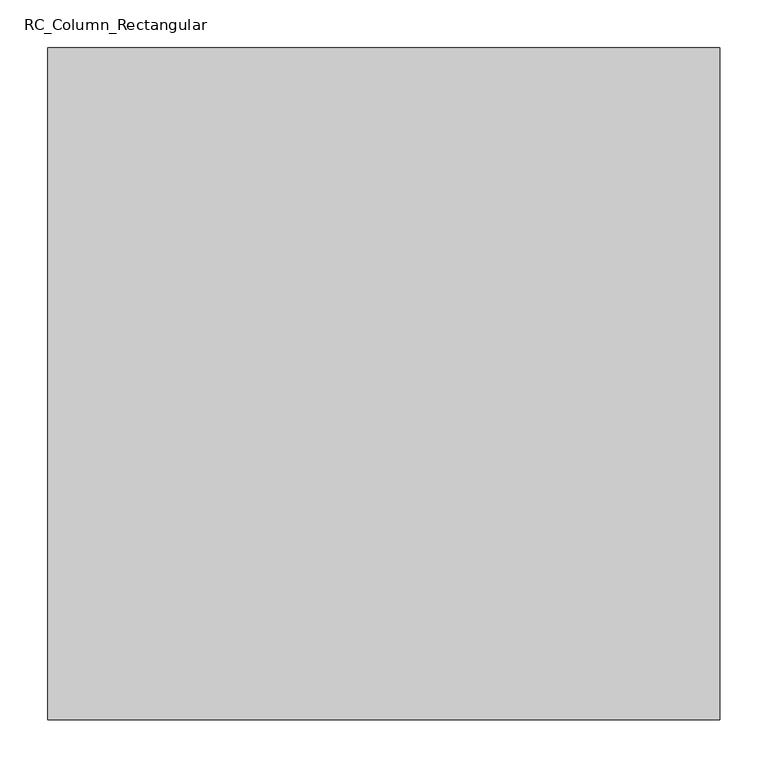
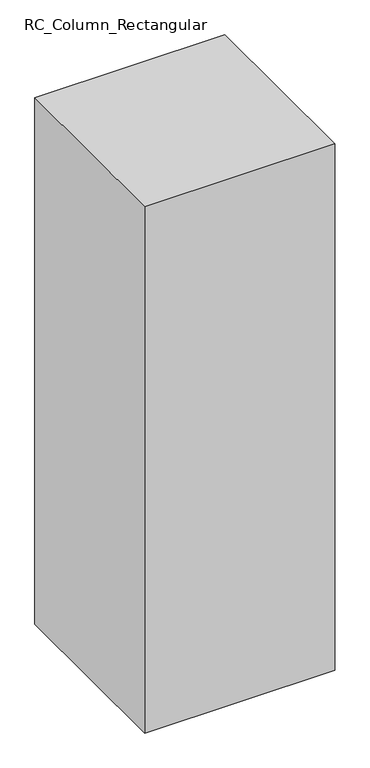
"""IFC4 building model written with IfcOpenShell, lengths in millimetres: column geometry, RC_Column_Rectangular : H_SC_AR_S15_UG PED_W700xL700_Bit_PD3."""

from ifc_helpers import new_model, si_unit, frame, origin, place, context, project, spatial, polyline, outline, extrude, source, transform, mapped, element, save


def rc_column_rectangular_f0532c4b(model_context):
    return source(origin(), model_context, "Body", "SweptSolid", [
        extrude(outline(polyline([(350.0, 350.0), (350.0, -350.0), (-350.0, -350.0), (-350.0, 350.0), (350.0, 350.0)])), frame((0.0, 0.0, -9380.1756499), z_axis=(0.0, 0.0, 1.0), x_axis=(1.0, 0.0, 0.0)), (0.0, 0.0, 1.0), 2050.0),
    ])


if __name__ == "__main__":
    model = new_model("IFC4")
    model_context = context("Model", 3, world=origin())
    ifc_project = project(units=[si_unit("LENGTHUNIT", "METRE", prefix="MILLI")], contexts=[model_context])
    site = spatial("IfcSite", under=ifc_project)
    building = spatial("IfcBuilding", under=site)
    placement = place(None, origin())
    rc_column_rectangular_shape = rc_column_rectangular_f0532c4b(model_context)
    element("IfcColumn", 1, ObjectType="RC_Column_Rectangular : H_SC_AR_S15_UG PED_W700xL700_Bit_PD3", at=placement, inside=building, context=model_context, shape_type="MappedRepresentation", body=[
        mapped(rc_column_rectangular_shape, transform((0.0, 0.0, 0.0), x_axis=(1.0, 0.0, 0.0), y_axis=(0.0, 1.0, 0.0), z_axis=(0.0, 0.0, 1.0))),
    ])
    save(model, "model.ifc")

# Revit data of these elements
# Type "RC_Column_Rectangular : H_SC_AR_S15_UG PED_W700xL700_Bit_PD3"
#   Type Mark = "PD3"
#   Width = 700 mm
#   Length = 700 mm
#   hec_material3 [instance default] = none
#   hec_material2 [instance default] = none
#   hec_material1 [instance default] = none
#   Structural Material [instance default] = none
#   Description = (empty or 0)
